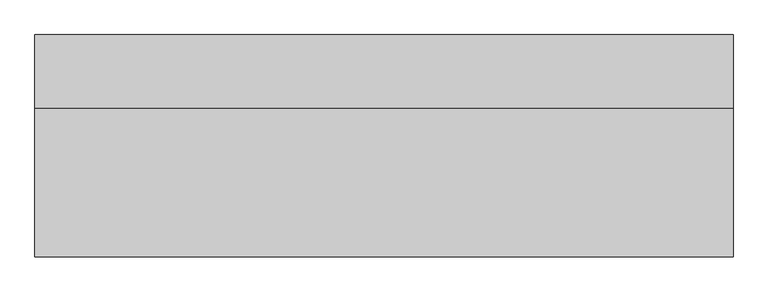
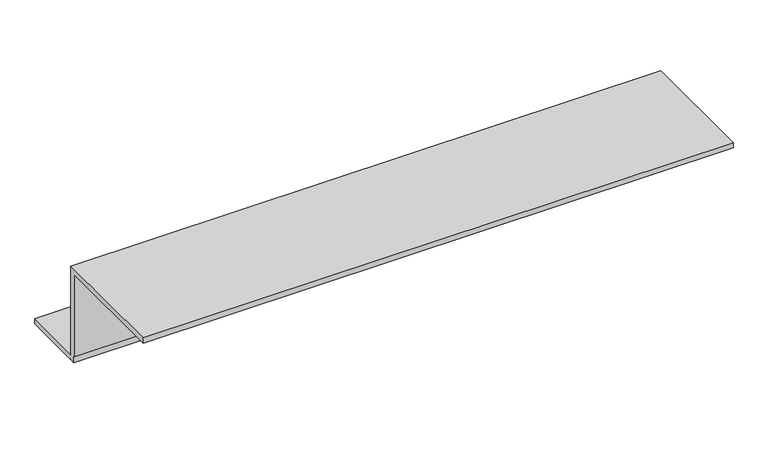
"""IFC4 building model written with IfcOpenShell, lengths in millimetres: proxy geometry, Stucco006 3383 : Stucco006 3383."""

from ifc_helpers import new_model, si_unit, frame, origin, place, context, project, spatial, polyline, outline, extrude, source, transform, mapped, element, save


def generic_models_24b3f6a2(model_context):
    return source(origin(), model_context, "Body", "SweptSolid", [
        extrude(outline(polyline([(10403.5368994, 39402.776), (10403.5368994, 39401.496), (10217.7209778, 39401.496), (10217.7209778, 39402.7319306), (10196.5677938, 39402.7319306), (10196.5677938, 39423.8851145), (10195.1623665, 39423.8851145), (10195.1623665, 39719.0425353), (9789.2215225, 39719.0425353), (9789.2215225, 39738.0484659), (10214.3377938, 39738.0484659), (10214.3377938, 39420.546875), (10425.9700834, 39420.546875), (10425.9700834, 39402.776), (10403.5368994, 39402.776)])), frame((3694.2883192, 0.0, 0.0), z_axis=(1.0, 0.0, 0.0), x_axis=(0.0, 1.0, 0.0)), (0.0, 0.0, 1.0), 2000.0),
    ])


if __name__ == "__main__":
    model = new_model("IFC4")
    model_context = context("Model", 3, world=origin())
    ifc_project = project(units=[si_unit("LENGTHUNIT", "METRE", prefix="MILLI")], contexts=[model_context])
    site = spatial("IfcSite", under=ifc_project)
    building = spatial("IfcBuilding", under=site)
    placement = place(None, origin())
    generic_models_shape = generic_models_24b3f6a2(model_context)
    element("IfcBuildingElementProxy", 1, Name="Stucco006 3383 : Stucco006 3383", ObjectType="Stucco006 3383 : Stucco006 3383", at=placement, inside=building, context=model_context, shape_type="MappedRepresentation", body=[
        mapped(generic_models_shape, transform((0.0, 0.0, 0.0), x_axis=(1.0, 0.0, 0.0), y_axis=(0.0, 1.0, 0.0), z_axis=(0.0, 0.0, 1.0))),
    ])
    save(model, "model.ifc")

# Revit data of these elements
# Type "Stucco006 3383 : Stucco006 3383"
#   NameOverride = "Stucco006"
# Element 1 (IfcBuildingElementProxy, "Stucco006 3383 : Stucco006 3383")
#   Materials on its faces: "7/8\" SMOOTH TROWEL EXTERIOR STUCCO"
# Materials
#   "7/8\" SMOOTH TROWEL EXTERIOR STUCCO": class "Unassigned", colour RGB 255 255 255, transparency 0, Cost = 0
